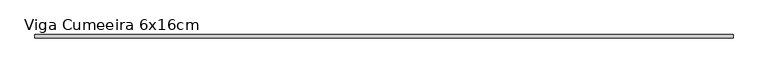
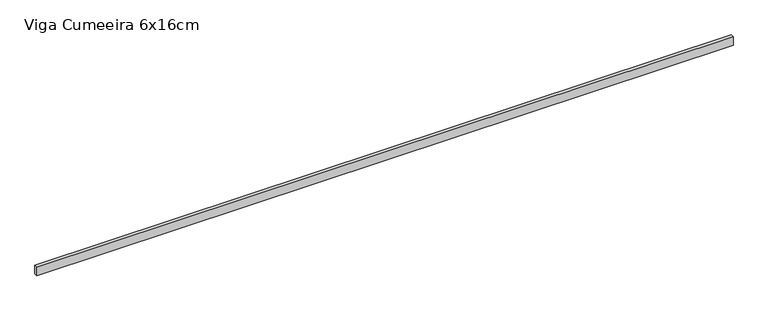
"""IFC4 building model written with IfcOpenShell, lengths in millimetres: beam geometry, Madeira de lei : Viga Cumeeira 6x16cm."""

import ifcopenshell
import ifcopenshell.guid

model = None  # the IFC model being written
_history = None  # IfcOwnerHistory: only IFC2X3 demands one
_inside = {}  # id of a spatial element -> (the spatial element, [elements in it])
_under = {}  # id of a project, library or spatial element -> (it, [spatial elements below it])
_declared = {}  # id of a project -> (the project, [libraries it declares])
_typed = {}  # id of a type object -> (the type object, [elements of that type])
_made_of = {}  # id of a material, layer set ... -> (it, [elements and type objects made of it])


def new_model(schema):
    """Start an empty IFC model of exactly this schema.

    Asked for "IFC4X3", IfcOpenShell would pick the latest addendum, in which some entities
    have other attributes; the version numbers below select the first issue.
    IFC2X3 requires an IfcOwnerHistory on every rooted entity: one is made here for all.
    """
    global model, _history
    if schema == "IFC4X3":
        model = ifcopenshell.file(schema_version=(4, 3, 0, 0))
    else:
        model = ifcopenshell.file(schema=schema)
    _inside.clear()
    _under.clear()
    _declared.clear()
    _typed.clear()
    _made_of.clear()
    _history = None
    if model.schema == "IFC2X3":
        org = make("IfcOrganization", Name="unknown")
        user = make(
            "IfcPersonAndOrganization",
            ThePerson=make("IfcPerson", FamilyName="unknown"),
            TheOrganization=org,
        )
        app = make(
            "IfcApplication",
            ApplicationDeveloper=org,
            Version="unknown",
            ApplicationFullName="unknown",
            ApplicationIdentifier="unknown",
        )
        _history = make(
            "IfcOwnerHistory",
            OwningUser=user,
            OwningApplication=app,
            ChangeAction="ADDED",
            CreationDate=0,
        )
    return model


def make(cls, **values):
    """One entity of the class cls with the attributes given. An attribute that is None is left unset."""
    return model.create_entity(
        cls, **{name: value for name, value in values.items() if value is not None}
    )


def rooted(cls, **values):
    """An entity with a GlobalId (a new one), such as an element, a storey or a relation."""
    return make(cls, GlobalId=ifcopenshell.guid.new(), OwnerHistory=_history, **values)


def si_unit(unit_type, name, prefix=None):
    """IfcSIUnit, for example si_unit("LENGTHUNIT", "METRE", prefix="MILLI")."""
    return make("IfcSIUnit", UnitType=unit_type, Prefix=prefix, Name=name)


def assignment(units):
    """IfcUnitAssignment: the units of a project."""
    return None if units is None else make("IfcUnitAssignment", Units=units)


def point(xyz):
    """IfcCartesianPoint."""
    return None if xyz is None else make("IfcCartesianPoint", Coordinates=xyz)


def direction(xyz):
    """IfcDirection."""
    return None if xyz is None else make("IfcDirection", DirectionRatios=xyz)


def frame(location, z_axis=None, x_axis=None):
    """IfcAxis2Placement3D, a coordinate frame: its origin and axes. An axis left out is left unset."""
    return make(
        "IfcAxis2Placement3D",
        Location=point(location),
        Axis=direction(z_axis),
        RefDirection=direction(x_axis),
    )


def origin():
    """The frame at (0, 0, 0) with its axes left unset."""
    return frame((0.0, 0.0, 0.0))


def place(relative_to, where):
    """IfcLocalPlacement: puts the frame where relative to a parent placement (None: the world)."""
    return make(
        "IfcLocalPlacement", PlacementRelTo=relative_to, RelativePlacement=where
    )


def context(
    kind, dimensions, precision=None, world=None, true_north=None, identifier=None
):
    """IfcGeometricRepresentationContext, for example the 3D "Model" context."""
    return make(
        "IfcGeometricRepresentationContext",
        ContextIdentifier=identifier,
        ContextType=kind,
        CoordinateSpaceDimension=dimensions,
        Precision=precision,
        WorldCoordinateSystem=world,
        TrueNorth=true_north,
    )


def project(units=None, contexts=None):
    """IfcProject with its units and contexts."""
    return rooted(
        "IfcProject",
        Name="project",
        RepresentationContexts=contexts,
        UnitsInContext=assignment(units),
    )


def spatial(cls, under=None, at=None, **own):
    """A site, building, storey or space (cls), placed at a placement, below another one or the project."""
    s = rooted(cls, ObjectPlacement=at, **own)
    if under is not None:
        _under.setdefault(under.id(), (under, []))[1].append(s)
    return s


def polyline(points):
    """IfcPolyline through the points."""
    return make("IfcPolyline", Points=[point(p) for p in points])


def outline(outer, holes=None, kind="AREA"):
    """IfcArbitraryClosedProfileDef: a profile drawn as a closed curve; with holes, ...WithVoids."""
    if holes is None:
        return make("IfcArbitraryClosedProfileDef", ProfileType=kind, OuterCurve=outer)
    return make(
        "IfcArbitraryProfileDefWithVoids",
        ProfileType=kind,
        OuterCurve=outer,
        InnerCurves=holes,
    )


def extrude(swept, where, along, depth):
    """IfcExtrudedAreaSolid: the profile swept, set in the frame where, extruded along a direction by depth."""
    return make(
        "IfcExtrudedAreaSolid",
        SweptArea=swept,
        Position=where,
        ExtrudedDirection=direction(along),
        Depth=depth,
    )


def shape(context_of_items, identifier, shape_type, items):
    """IfcShapeRepresentation: the items that make up one representation, for example the "Body"."""
    return make(
        "IfcShapeRepresentation",
        ContextOfItems=context_of_items,
        RepresentationIdentifier=identifier,
        RepresentationType=shape_type,
        Items=items,
    )


def source(mapping_origin, context_of_items, identifier, shape_type, items):
    """IfcRepresentationMap: a shape defined once, which mapped items show again and again."""
    return make(
        "IfcRepresentationMap",
        MappingOrigin=mapping_origin,
        MappedRepresentation=shape(context_of_items, identifier, shape_type, items),
    )


def transform(
    local_origin,
    x_axis=None,
    y_axis=None,
    z_axis=None,
    scale=None,
    scale2=None,
    scale3=None,
    uniform=True,
):
    """IfcCartesianTransformationOperator3D, or its non-uniform kind. x_axis, y_axis, z_axis: its Axis1, 2, 3."""
    if uniform:
        return make(
            "IfcCartesianTransformationOperator3D",
            Axis1=direction(x_axis),
            Axis2=direction(y_axis),
            LocalOrigin=point(local_origin),
            Scale=scale,
            Axis3=direction(z_axis),
        )
    return make(
        "IfcCartesianTransformationOperator3DnonUniform",
        Axis1=direction(x_axis),
        Axis2=direction(y_axis),
        LocalOrigin=point(local_origin),
        Scale=scale,
        Axis3=direction(z_axis),
        Scale2=scale2,
        Scale3=scale3,
    )


def mapped(mapping_source, mapping_target):
    """IfcMappedItem: shows the shape of a source again, moved by a transform."""
    return make(
        "IfcMappedItem", MappingSource=mapping_source, MappingTarget=mapping_target
    )


def made_of(thing, what):
    """Note that an element or type object is made of a material, layer set ...; save() writes the relation."""
    if what is not None:
        _made_of.setdefault(what.id(), (what, []))[1].append(thing)
    return thing


def element(
    cls,
    number,
    at=None,
    inside=None,
    cuts=None,
    type_object=None,
    material=None,
    context=None,
    identifier="Body",
    shape_type=None,
    held_by="IfcProductDefinitionShape",
    body=None,
    shapes=None,
    **own,
):
    """One element of the class cls, such as IfcWall. Its Tag is "e" and its number.

    at: its placement. inside: the storey or other place that contains it. cuts: it is an
    opening in that element (IfcRelVoidsElement). A single representation is given by context,
    identifier, shape_type and body (its items); several are given by shapes. held_by: the class
    of the entity that holds the representations. save() writes the other relations.
    """
    e = rooted(cls, Tag="e%d" % number, ObjectPlacement=at, **own)
    if body is not None:
        shapes = [shape(context, identifier, shape_type, body)]
    if shapes is not None:
        e.Representation = make(held_by, Representations=shapes)
    if inside is not None:
        _inside.setdefault(inside.id(), (inside, []))[1].append(e)
    if cuts is not None:
        rooted(
            "IfcRelVoidsElement", RelatingBuildingElement=cuts, RelatedOpeningElement=e
        )
    if type_object is not None:
        _typed.setdefault(type_object.id(), (type_object, []))[1].append(e)
    return made_of(e, material)


def aggregate(whole, parts):
    """IfcRelAggregates: a whole, such as a stair, and the parts it consists of."""
    return rooted("IfcRelAggregates", RelatingObject=whole, RelatedObjects=parts)


def save(model, path):
    """Write the relations noted so far, then the file.

    IfcRelAggregates (storeys below a building ...), IfcRelContainedInSpatialStructure (elements
    in a storey), IfcRelDefinesByType, IfcRelAssociatesMaterial and IfcRelDeclares: one each for
    every whole, place, type object, material and project.
    """
    for whole, parts in _under.values():
        aggregate(whole, parts)
    for where, things in _inside.values():
        rooted(
            "IfcRelContainedInSpatialStructure",
            RelatedElements=things,
            RelatingStructure=where,
        )
    for kind, things in _typed.values():
        rooted("IfcRelDefinesByType", RelatedObjects=things, RelatingType=kind)
    for what, things in _made_of.values():
        rooted("IfcRelAssociatesMaterial", RelatedObjects=things, RelatingMaterial=what)
    for by, libraries in _declared.values():
        rooted("IfcRelDeclares", RelatingContext=by, RelatedDefinitions=libraries)
    model.write(path)


def viga_cumeeira_6x16cm_b61bb166(model_context):
    return source(origin(), model_context, "Body", "SweptSolid", [
        extrude(outline(polyline([(6210.0, 30.0), (6210.0, -30.0), (-6210.0, -30.0), (-6210.0, 30.0), (6210.0, 30.0)])), frame((0.0, 0.0, -80.0), z_axis=(0.0, 0.0, 1.0), x_axis=(1.0, 0.0, 0.0)), (0.0, 0.0, 1.0), 160.0),
    ])


if __name__ == "__main__":
    model = new_model("IFC4")
    model_context = context("Model", 3, world=origin())
    ifc_project = project(units=[si_unit("LENGTHUNIT", "METRE", prefix="MILLI")], contexts=[model_context])
    site = spatial("IfcSite", under=ifc_project)
    building = spatial("IfcBuilding", under=site)
    placement = place(None, origin())
    viga_cumeeira_6x16cm_shape = viga_cumeeira_6x16cm_b61bb166(model_context)
    element("IfcBeam", 1, ObjectType="Madeira de lei : Viga Cumeeira 6x16cm", at=placement, inside=building, context=model_context, shape_type="MappedRepresentation", body=[
        mapped(viga_cumeeira_6x16cm_shape, transform((0.0, 0.0, 0.0), x_axis=(1.0, 0.0, 0.0), y_axis=(0.0, 1.0, 0.0), z_axis=(0.0, 0.0, 1.0))),
    ])
    save(model, "model.ifc")

# Revit data of these elements
# Type "Madeira de lei : Viga Cumeeira 6x16cm"
#   A = 0.02 m²
#   Length [instance default] = 1.524 m
#   b = 0.06 m
#   d = 0.16 m
#   Structural Material [instance default] = none
#   Assembly Code = ""
# Element 1 (IfcBeam, "Madeira de lei : Viga Cumeeira 6x16cm")
#   Structural Material = .MADEIRAMENTO
#   Materials on its faces: ".MADEIRAMENTO"
# Materials
#   ".MADEIRAMENTO": class ".CC_MADEIRAS", colour RGB 212 179 113, transparency 0, Cost = 0
